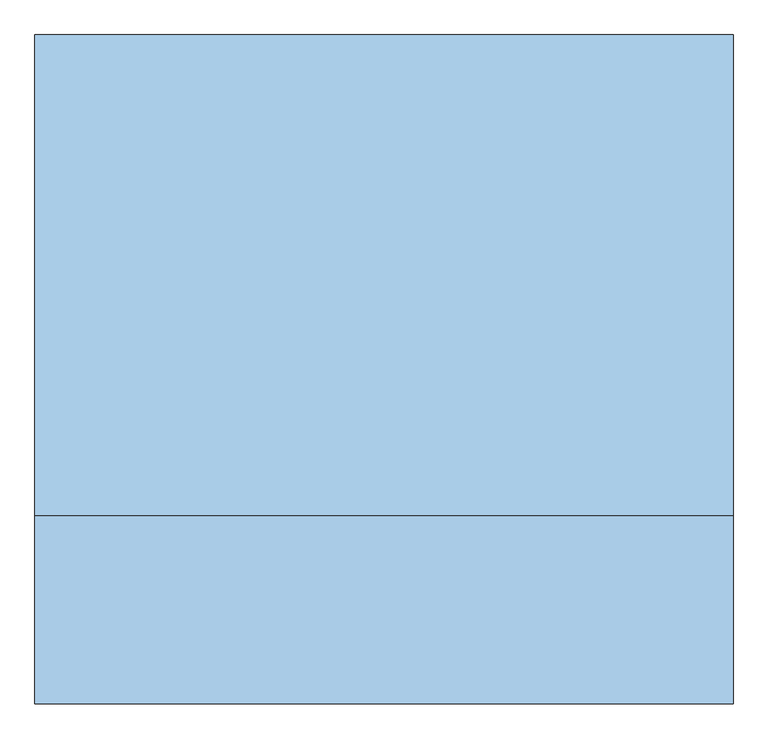
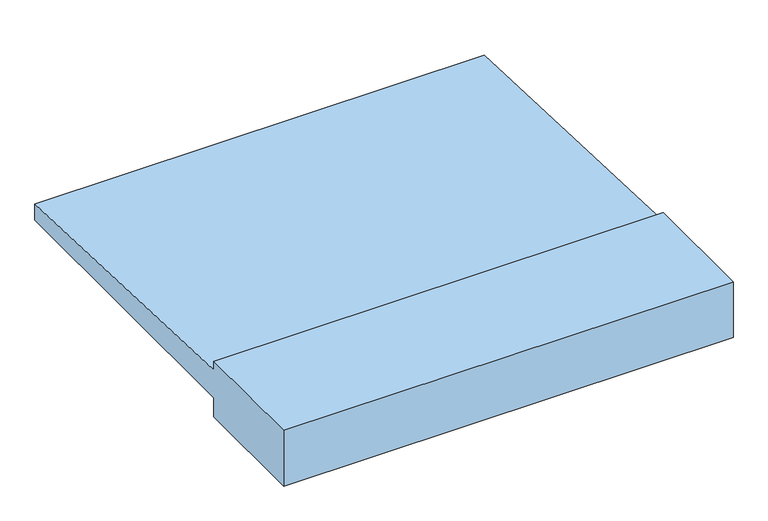
"""IFC4 building model written with IfcOpenShell, lengths in millimetres: window geometry, 캐노피 : 캐노피."""

from ifc_helpers import new_model, si_unit, frame, origin, place, context, project, spatial, polyline, outline, extrude, source, transform, mapped, element, save


def window_1abda111(model_context):
    return source(origin(), model_context, "Body", "SweptSolid", [
        extrude(outline(polyline([(-195.0, 800.0), (-195.0, 990.0), (195.0, 990.0), (195.0, 960.0), (1195.0, 920.0), (1195.0, 865.0), (195.0, 865.0), (195.0, 800.0), (-195.0, 800.0)])), frame((-725.0, 0.0, 0.0), z_axis=(1.0, 0.0, 0.0), x_axis=(0.0, 1.0, 0.0)), (0.0, 0.0, 1.0), 1450.0),
    ])


if __name__ == "__main__":
    model = new_model("IFC4")
    model_context = context("Model", 3, world=origin())
    ifc_project = project(units=[si_unit("LENGTHUNIT", "METRE", prefix="MILLI")], contexts=[model_context])
    site = spatial("IfcSite", under=ifc_project)
    building = spatial("IfcBuilding", under=site)
    placement = place(None, origin())
    window_shape = window_1abda111(model_context)
    element("IfcWindow", 1, ObjectType="캐노피 : 캐노피", at=placement, inside=building, context=model_context, shape_type="MappedRepresentation", body=[
        mapped(window_shape, transform((0.0, 0.0, 0.0), x_axis=(1.0, 0.0, 0.0), y_axis=(0.0, 1.0, 0.0), z_axis=(0.0, 0.0, 1.0))),
    ])
    save(model, "model.ifc")

# Revit data of these elements
# Type "캐노피 : 캐노피"
#   Type Mark = "203"
#   돌출길이 = 1000 mm
#   Height = 190 mm
#   Default Sill Height = 800 mm
#   Width = 1450 mm
#   Wall Closure = (empty or 0)
